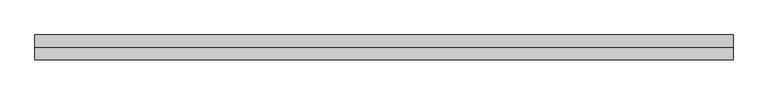
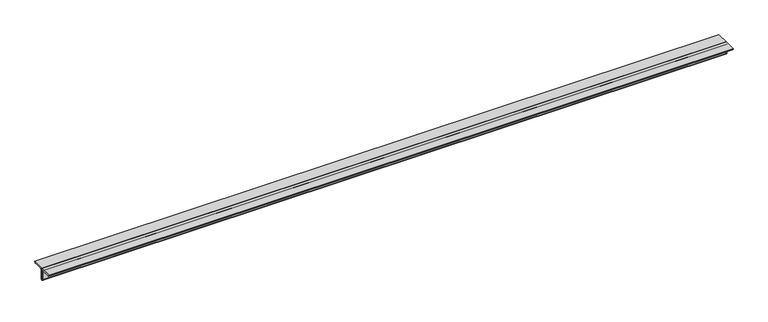
"""IFC4 building model written with IfcOpenShell, lengths in millimetres: member geometry, Steel Framing_2Ls_KS : H_SB_AR_S02_2Ls-100x100x10_VBR1."""

from ifc_helpers import new_model, si_unit, point, frame, frame_2d, origin, place, context, project, spatial, polyline, circle_curve, trimmed, segment, composite_curve, outline, extrude, source, transform, mapped, element, save


def member_a0fa3de0(model_context):
    return source(origin(), model_context, "Body", "SweptSolid", [
        extrude(outline(composite_curve([segment(polyline([(0.0, 28.2), (100.0, 28.2)]), True, "CONTINUOUS"), segment(trimmed(circle_curve(frame_2d((90.0, 28.2)), 10.0), [point((100.0, 28.2))], [point((90.0, 18.2))], False, "CARTESIAN"), True, "CONTINUOUS"), segment(polyline([(90.0, 18.2), (20.0, 18.2)]), True, "CONTINUOUS"), segment(trimmed(circle_curve(frame_2d((20.0, 8.2)), 10.0), [point((20.0, 18.2))], [point((10.0, 8.2))], True, "CARTESIAN"), True, "CONTINUOUS"), segment(polyline([(10.0, 8.2), (10.0, -61.8)]), True, "CONTINUOUS"), segment(trimmed(circle_curve(frame_2d((0.0, -61.8)), 10.0), [point((10.0, -61.8))], [point((0.0, -71.8))], False, "CARTESIAN"), True, "CONTINUOUS"), segment(polyline([(0.0, -71.8), (0.0, 28.2)]), True, "CONTINUOUS")], self_intersect=False)), frame((-2842.7759474, 0.0, 0.0), z_axis=(1.0, 0.0, 0.0), x_axis=(0.0, 1.0, 0.0)), (0.0, 0.0, 1.0), 5598.0876164),
        extrude(outline(composite_curve([segment(polyline([(0.0, 28.2), (0.0, -71.8)]), True, "CONTINUOUS"), segment(trimmed(circle_curve(frame_2d((0.0, -61.8)), 10.0), [point((0.0, -71.8))], [point((-10.0, -61.8))], False, "CARTESIAN"), True, "CONTINUOUS"), segment(polyline([(-10.0, -61.8), (-10.0, 8.2)]), True, "CONTINUOUS"), segment(trimmed(circle_curve(frame_2d((-20.0, 8.2)), 10.0), [point((-10.0, 8.2))], [point((-20.0, 18.2))], True, "CARTESIAN"), True, "CONTINUOUS"), segment(polyline([(-20.0, 18.2), (-90.0, 18.2)]), True, "CONTINUOUS"), segment(trimmed(circle_curve(frame_2d((-90.0, 28.2)), 10.0), [point((-90.0, 18.2))], [point((-100.0, 28.2))], False, "CARTESIAN"), True, "CONTINUOUS"), segment(polyline([(-100.0, 28.2), (0.0, 28.2)]), True, "CONTINUOUS")], self_intersect=False)), frame((-2842.7759474, 0.0, 0.0), z_axis=(1.0, 0.0, 0.0), x_axis=(0.0, 1.0, 0.0)), (0.0, 0.0, 1.0), 5598.0876164),
    ])


if __name__ == "__main__":
    model = new_model("IFC4")
    model_context = context("Model", 3, world=origin())
    ifc_project = project(units=[si_unit("LENGTHUNIT", "METRE", prefix="MILLI")], contexts=[model_context])
    site = spatial("IfcSite", under=ifc_project)
    building = spatial("IfcBuilding", under=site)
    placement = place(None, origin())
    member_shape = member_a0fa3de0(model_context)
    element("IfcMember", 1, ObjectType="Steel Framing_2Ls_KS : H_SB_AR_S02_2Ls-100x100x10_VBR1", at=placement, inside=building, context=model_context, shape_type="MappedRepresentation", body=[
        mapped(member_shape, transform((0.0, 0.0, 0.0), x_axis=(1.0, 0.0, 0.0), y_axis=(0.0, 1.0, 0.0), z_axis=(0.0, 0.0, 1.0))),
    ])
    save(model, "model.ifc")

# Revit data of these elements
# Type "Steel Framing_2Ls_KS : H_SB_AR_S02_2Ls-100x100x10_VBR1"
#   Type Comments = "MAIN"
#   Type Mark = "VBR1"
#   H_SectionID = "2Ls-100x100x10"
#   Assembly Code = "B10"
#   Legs = "LLBB"
#   H_Ratio for Additional Steel Plate = 0.2
#   W = 0
#   Perimeter = 0.80 m²/m
#   Nominal Weight = 29.80 kgf/m
#   Length [instance default] = 1524 mm
#   Space = 0 mm
#   b = 100 mm
#   d = 100 mm
#   t = 10 mm
#   y = 28.2 mm
#   A = 0.0038 m²
#   Structural Material [instance default] = Steel, 45-345
# Element 1 (IfcMember, "Steel Framing_2Ls_KS : H_SB_AR_S02_2Ls-100x100x10_VBR1")
#   Materials on its faces: "Steel, 45-345"
# Materials
#   "Steel, 45-345": class "Metal", colour RGB 189 187 185, transparency 0, Description = "Steel 345 MPa", Cost = 0
